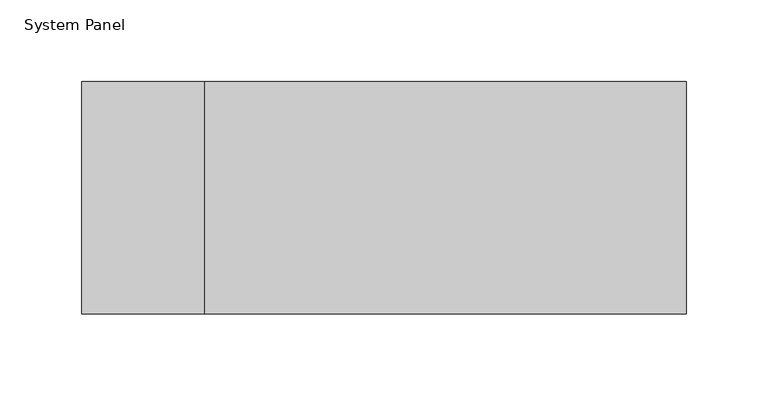
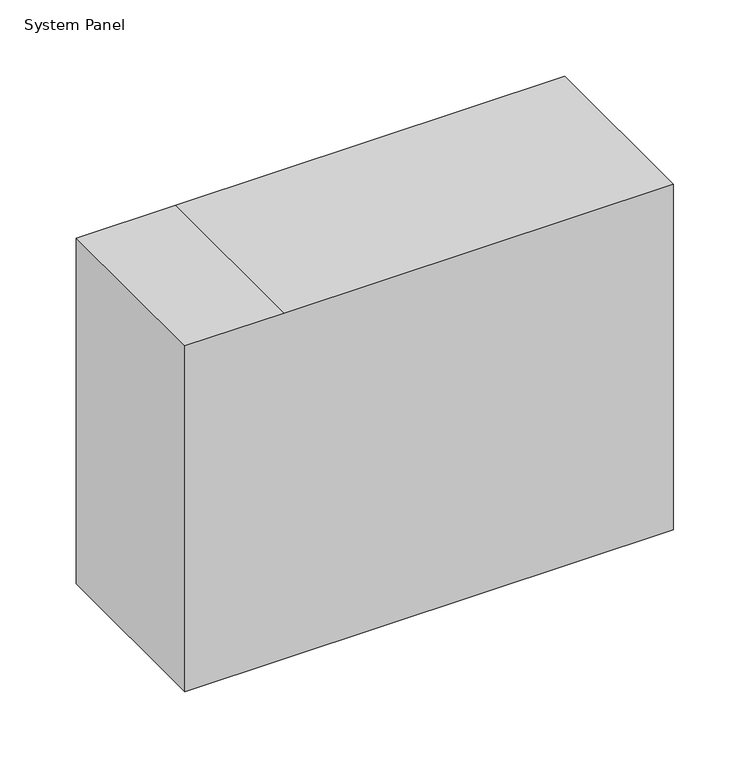
"""IFC4 building model written with IfcOpenShell, lengths in millimetres: plate geometry, System Panel : NLRS_21_CWP_hsb-vulling minerale wol 142 _gen_rsf."""

from ifc_helpers import new_model, si_unit, frame, origin, place, context, project, spatial, polyline, outline, extrude, source, transform, mapped, element, save


def system_panel_37dbae85(model_context):
    return source(origin(), model_context, "Body", "SweptSolid", [
        extrude(outline(polyline([(0.0, -184.5), (0.0, -109.3441061), (0.0, 184.5), (276.0, 184.5), (276.0, -109.3441061), (276.0, -184.5), (0.0, -184.5)])), frame((0.0, -71.0, 0.0), z_axis=(0.0, 1.0, 0.0), x_axis=(0.0, 0.0, 1.0)), (0.0, 0.0, 1.0), 142.0),
    ])


if __name__ == "__main__":
    model = new_model("IFC4")
    model_context = context("Model", 3, world=origin())
    ifc_project = project(units=[si_unit("LENGTHUNIT", "METRE", prefix="MILLI")], contexts=[model_context])
    site = spatial("IfcSite", under=ifc_project)
    building = spatial("IfcBuilding", under=site)
    placement = place(None, origin())
    system_panel_shape = system_panel_37dbae85(model_context)
    element("IfcPlate", 1, ObjectType="System Panel : NLRS_21_CWP_hsb-vulling minerale wol 142 _gen_rsf", at=placement, inside=building, context=model_context, shape_type="MappedRepresentation", body=[
        mapped(system_panel_shape, transform((0.0, 0.0, 0.0), x_axis=(1.0, 0.0, 0.0), y_axis=(0.0, 1.0, 0.0), z_axis=(0.0, 0.0, 1.0))),
    ])
    save(model, "model.ifc")

# Revit data of these elements
# Type "System Panel : NLRS_21_CWP_hsb-vulling minerale wol 142 _gen_rsf"
#   Export Type to IFC As = "IfcWall"
#   Type IfcGUID = "07M7mRoiH1CR8m_RSKIwpC"
#   Assembly Code = "21.23"
# Element 1 (IfcPlate, "System Panel : NLRS_21_CWP_hsb-vulling minerale wol 142 _gen_rsf")
#   Materials on its faces: "NLRS_m1_isolatie minerale wol_gen_rsf"
# Materials
#   "NLRS_m1_isolatie minerale wol_gen_rsf": class "M - Anorganische materialen", colour RGB 200 200 140, transparency 0, Keynote = "m1", Manufacturer = "Revit Standards Foundation", URL = "www.revitstandards.org", Description = "isolatie minerale wol", Cost = 0
